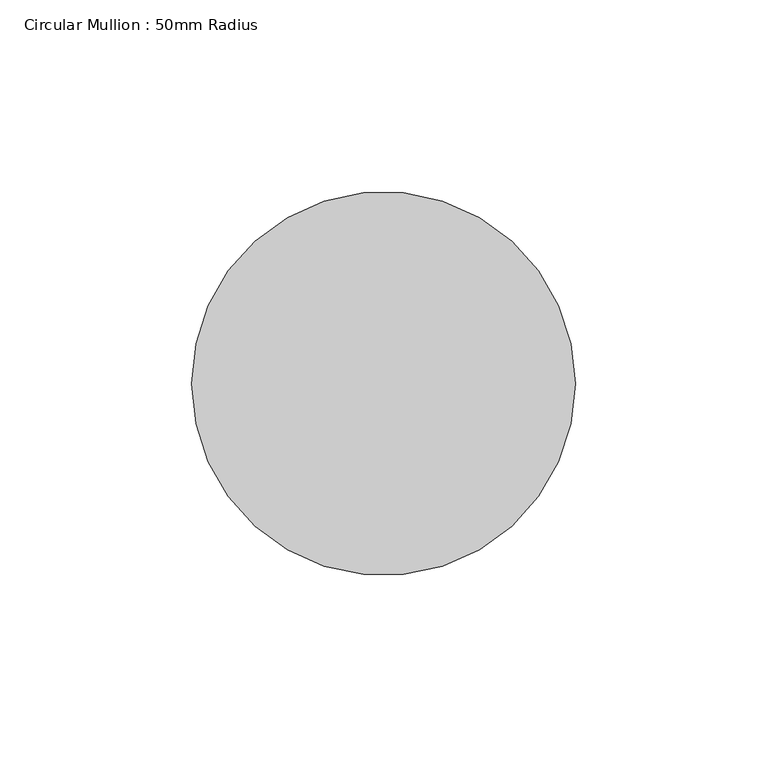
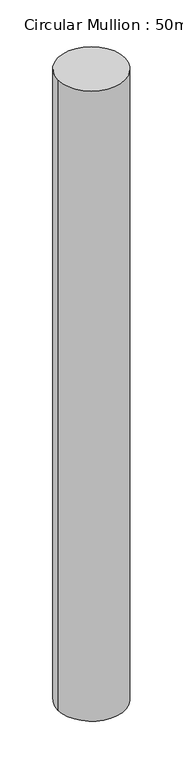
"""IFC4 building model written with IfcOpenShell, lengths in millimetres: member geometry, Circular Mullion : 50mm Radius."""

from ifc_helpers import new_model, si_unit, point, frame, origin, origin_2d, place, context, project, spatial, circle_curve, trimmed, segment, composite_curve, outline, extrude, source, transform, mapped, element, save


def circular_mullion_50mm_radius_97294470(model_context):
    return source(origin(), model_context, "Body", "SweptSolid", [
        extrude(outline(composite_curve([segment(trimmed(circle_curve(origin_2d(), 50.0), [point((50.0, 0.0))], [point((-50.0, 0.0))], False, "CARTESIAN"), True, "CONTINUOUS"), segment(trimmed(circle_curve(origin_2d(), 50.0), [point((-50.0, 0.0))], [point((50.0, 0.0))], False, "CARTESIAN"), True, "CONTINUOUS")], self_intersect=False)), frame((0.0, 0.0, -995.5194694), z_axis=(0.0, 0.0, 1.0), x_axis=(1.0, 0.0, 0.0)), (0.0, 0.0, 1.0), 995.5194694),
    ])


if __name__ == "__main__":
    model = new_model("IFC4")
    model_context = context("Model", 3, world=origin())
    ifc_project = project(units=[si_unit("LENGTHUNIT", "METRE", prefix="MILLI")], contexts=[model_context])
    site = spatial("IfcSite", under=ifc_project)
    building = spatial("IfcBuilding", under=site)
    placement = place(None, origin())
    circular_mullion_50mm_radius_shape = circular_mullion_50mm_radius_97294470(model_context)
    element("IfcMember", 1, ObjectType="Circular Mullion : 50mm Radius", at=placement, inside=building, context=model_context, shape_type="MappedRepresentation", body=[
        mapped(circular_mullion_50mm_radius_shape, transform((0.0, 0.0, 0.0), x_axis=(1.0, 0.0, 0.0), y_axis=(0.0, 1.0, 0.0), z_axis=(0.0, 0.0, 1.0))),
    ])
    save(model, "model.ifc")

# Revit data of these elements
# Type "Circular Mullion : 50mm Radius"
#   built-in parameter 1007350 = 0.164042 (stored number, unit not read)
# Element 1 (IfcMember, "Circular Mullion : 50mm Radius")
#   Materials on its faces: "Aluminium"
# Materials
#   "Aluminium": class "Metal", colour RGB 247 247 247, transparency 0, Description = "Aluminium 6061", Cost = 0
